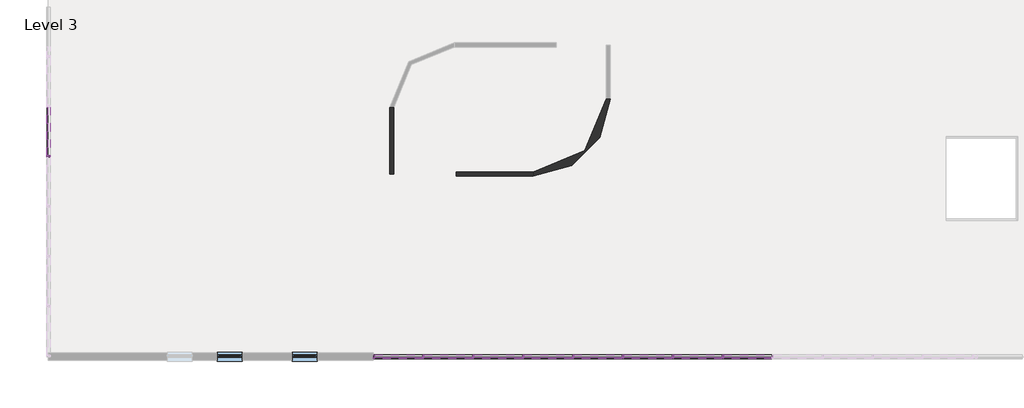
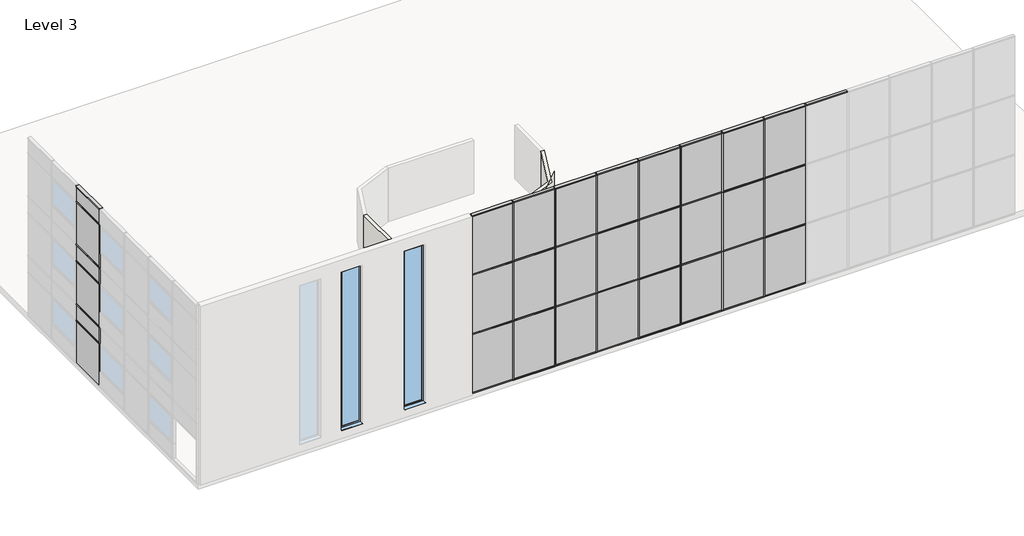
# One storey, part 2 of 5: 69 members, 30 plates, 3 walls, 2 windows.
"""IFC4 building model written with IfcOpenShell, lengths in millimetres."""

import ifcopenshell
import ifcopenshell.guid

model = None  # the IFC model being written
_history = None  # IfcOwnerHistory: only IFC2X3 demands one
_inside = {}  # id of a spatial element -> (the spatial element, [elements in it])
_under = {}  # id of a project, library or spatial element -> (it, [spatial elements below it])
_declared = {}  # id of a project -> (the project, [libraries it declares])
_typed = {}  # id of a type object -> (the type object, [elements of that type])
_made_of = {}  # id of a material, layer set ... -> (it, [elements and type objects made of it])


def new_model(schema):
    """Start an empty IFC model of exactly this schema.

    Asked for "IFC4X3", IfcOpenShell would pick the latest addendum, in which some entities
    have other attributes; the version numbers below select the first issue.
    IFC2X3 requires an IfcOwnerHistory on every rooted entity: one is made here for all.
    """
    global model, _history
    if schema == "IFC4X3":
        model = ifcopenshell.file(schema_version=(4, 3, 0, 0))
    else:
        model = ifcopenshell.file(schema=schema)
    _inside.clear()
    _under.clear()
    _declared.clear()
    _typed.clear()
    _made_of.clear()
    _history = None
    if model.schema == "IFC2X3":
        org = make("IfcOrganization", Name="unknown")
        user = make(
            "IfcPersonAndOrganization",
            ThePerson=make("IfcPerson", FamilyName="unknown"),
            TheOrganization=org,
        )
        app = make(
            "IfcApplication",
            ApplicationDeveloper=org,
            Version="unknown",
            ApplicationFullName="unknown",
            ApplicationIdentifier="unknown",
        )
        _history = make(
            "IfcOwnerHistory",
            OwningUser=user,
            OwningApplication=app,
            ChangeAction="ADDED",
            CreationDate=0,
        )
    return model


def make(cls, **values):
    """One entity of the class cls with the attributes given. An attribute that is None is left unset."""
    return model.create_entity(
        cls, **{name: value for name, value in values.items() if value is not None}
    )


def rooted(cls, **values):
    """An entity with a GlobalId (a new one), such as an element, a storey or a relation."""
    return make(cls, GlobalId=ifcopenshell.guid.new(), OwnerHistory=_history, **values)


def si_unit(unit_type, name, prefix=None):
    """IfcSIUnit, for example si_unit("LENGTHUNIT", "METRE", prefix="MILLI")."""
    return make("IfcSIUnit", UnitType=unit_type, Prefix=prefix, Name=name)


def assignment(units):
    """IfcUnitAssignment: the units of a project."""
    return None if units is None else make("IfcUnitAssignment", Units=units)


def point(xyz):
    """IfcCartesianPoint."""
    return None if xyz is None else make("IfcCartesianPoint", Coordinates=xyz)


def direction(xyz):
    """IfcDirection."""
    return None if xyz is None else make("IfcDirection", DirectionRatios=xyz)


def frame(location, z_axis=None, x_axis=None):
    """IfcAxis2Placement3D, a coordinate frame: its origin and axes. An axis left out is left unset."""
    return make(
        "IfcAxis2Placement3D",
        Location=point(location),
        Axis=direction(z_axis),
        RefDirection=direction(x_axis),
    )


def frame_2d(location, x_axis=None):
    """IfcAxis2Placement2D, a coordinate frame in the plane: its origin and x axis."""
    return make(
        "IfcAxis2Placement2D", Location=point(location), RefDirection=direction(x_axis)
    )


def origin():
    """The frame at (0, 0, 0) with its axes left unset."""
    return frame((0.0, 0.0, 0.0))


def origin_with_axes():
    """The frame at (0, 0, 0) with the z axis (0, 0, 1) and the x axis (1, 0, 0) written out."""
    return frame((0.0, 0.0, 0.0), z_axis=(0.0, 0.0, 1.0), x_axis=(1.0, 0.0, 0.0))


def place(relative_to, where):
    """IfcLocalPlacement: puts the frame where relative to a parent placement (None: the world)."""
    return make(
        "IfcLocalPlacement", PlacementRelTo=relative_to, RelativePlacement=where
    )


def context(
    kind, dimensions, precision=None, world=None, true_north=None, identifier=None
):
    """IfcGeometricRepresentationContext, for example the 3D "Model" context."""
    return make(
        "IfcGeometricRepresentationContext",
        ContextIdentifier=identifier,
        ContextType=kind,
        CoordinateSpaceDimension=dimensions,
        Precision=precision,
        WorldCoordinateSystem=world,
        TrueNorth=true_north,
    )


def project(units=None, contexts=None):
    """IfcProject with its units and contexts."""
    return rooted(
        "IfcProject",
        Name="project",
        RepresentationContexts=contexts,
        UnitsInContext=assignment(units),
    )


def spatial(cls, under=None, at=None, **own):
    """A site, building, storey or space (cls), placed at a placement, below another one or the project."""
    s = rooted(cls, ObjectPlacement=at, **own)
    if under is not None:
        _under.setdefault(under.id(), (under, []))[1].append(s)
    return s


def polyline(points):
    """IfcPolyline through the points."""
    return make("IfcPolyline", Points=[point(p) for p in points])


def circle_curve(where, radius):
    """IfcCircle in the frame where."""
    return make("IfcCircle", Position=where, Radius=radius)


def trimmed(basis, trim1, trim2, sense, master):
    """IfcTrimmedCurve: the piece of a basis curve between two trims."""
    return make(
        "IfcTrimmedCurve",
        BasisCurve=basis,
        Trim1=trim1,
        Trim2=trim2,
        SenseAgreement=sense,
        MasterRepresentation=master,
    )


def segment(curve, same_sense, transition):
    """IfcCompositeCurveSegment."""
    return make(
        "IfcCompositeCurveSegment",
        Transition=transition,
        SameSense=same_sense,
        ParentCurve=curve,
    )


def composite_curve(segments, self_intersect=None):
    """IfcCompositeCurve: segments joined end to end."""
    return make("IfcCompositeCurve", Segments=segments, SelfIntersect=self_intersect)


def outline(outer, holes=None, kind="AREA"):
    """IfcArbitraryClosedProfileDef: a profile drawn as a closed curve; with holes, ...WithVoids."""
    if holes is None:
        return make("IfcArbitraryClosedProfileDef", ProfileType=kind, OuterCurve=outer)
    return make(
        "IfcArbitraryProfileDefWithVoids",
        ProfileType=kind,
        OuterCurve=outer,
        InnerCurves=holes,
    )


def extrude(swept, where, along, depth):
    """IfcExtrudedAreaSolid: the profile swept, set in the frame where, extruded along a direction by depth."""
    return make(
        "IfcExtrudedAreaSolid",
        SweptArea=swept,
        Position=where,
        ExtrudedDirection=direction(along),
        Depth=depth,
    )


def faces_of(points, faces, orient=None, outer=None):
    """IfcFace entities. A face is a list of loops; a loop is a list of indices into points, from 0.

    orient and outer hold one flag for each loop. By default every Orientation is true, the
    first loop of a face is its IfcFaceOuterBound and the others are IfcFaceBound.
    """
    made = []
    for i, loops in enumerate(faces):
        bounds = []
        for j, loop in enumerate(loops):
            is_outer = j == 0 if outer is None else outer[i][j]
            bounds.append(
                make(
                    "IfcFaceOuterBound" if is_outer else "IfcFaceBound",
                    Bound=make("IfcPolyLoop", Polygon=[points[k] for k in loop]),
                    Orientation=True if orient is None else orient[i][j],
                )
            )
        made.append(make("IfcFace", Bounds=bounds))
    return made


def faceted_brep(points, faces, orient=None, outer=None, voids=None):
    """IfcFacetedBrep: a solid bounded by flat faces; with voids (closed shells), ...WithVoids."""
    shared = [point(p) for p in points]
    hull = make("IfcClosedShell", CfsFaces=faces_of(shared, faces, orient, outer))
    if voids is None:
        return make("IfcFacetedBrep", Outer=hull)
    return make(
        "IfcFacetedBrepWithVoids",
        Outer=hull,
        Voids=[
            make(cls, CfsFaces=faces_of(shared, fs, o, b)) for cls, fs, o, b in voids
        ],
    )


def shape(context_of_items, identifier, shape_type, items):
    """IfcShapeRepresentation: the items that make up one representation, for example the "Body"."""
    return make(
        "IfcShapeRepresentation",
        ContextOfItems=context_of_items,
        RepresentationIdentifier=identifier,
        RepresentationType=shape_type,
        Items=items,
    )


def source(mapping_origin, context_of_items, identifier, shape_type, items):
    """IfcRepresentationMap: a shape defined once, which mapped items show again and again."""
    return make(
        "IfcRepresentationMap",
        MappingOrigin=mapping_origin,
        MappedRepresentation=shape(context_of_items, identifier, shape_type, items),
    )


def transform(
    local_origin,
    x_axis=None,
    y_axis=None,
    z_axis=None,
    scale=None,
    scale2=None,
    scale3=None,
    uniform=True,
):
    """IfcCartesianTransformationOperator3D, or its non-uniform kind. x_axis, y_axis, z_axis: its Axis1, 2, 3."""
    if uniform:
        return make(
            "IfcCartesianTransformationOperator3D",
            Axis1=direction(x_axis),
            Axis2=direction(y_axis),
            LocalOrigin=point(local_origin),
            Scale=scale,
            Axis3=direction(z_axis),
        )
    return make(
        "IfcCartesianTransformationOperator3DnonUniform",
        Axis1=direction(x_axis),
        Axis2=direction(y_axis),
        LocalOrigin=point(local_origin),
        Scale=scale,
        Axis3=direction(z_axis),
        Scale2=scale2,
        Scale3=scale3,
    )


def mapped(mapping_source, mapping_target):
    """IfcMappedItem: shows the shape of a source again, moved by a transform."""
    return make(
        "IfcMappedItem", MappingSource=mapping_source, MappingTarget=mapping_target
    )


def made_of(thing, what):
    """Note that an element or type object is made of a material, layer set ...; save() writes the relation."""
    if what is not None:
        _made_of.setdefault(what.id(), (what, []))[1].append(thing)
    return thing


def element(
    cls,
    number,
    at=None,
    inside=None,
    cuts=None,
    type_object=None,
    material=None,
    context=None,
    identifier="Body",
    shape_type=None,
    held_by="IfcProductDefinitionShape",
    body=None,
    shapes=None,
    **own,
):
    """One element of the class cls, such as IfcWall. Its Tag is "e" and its number.

    at: its placement. inside: the storey or other place that contains it. cuts: it is an
    opening in that element (IfcRelVoidsElement). A single representation is given by context,
    identifier, shape_type and body (its items); several are given by shapes. held_by: the class
    of the entity that holds the representations. save() writes the other relations.
    """
    e = rooted(cls, Tag="e%d" % number, ObjectPlacement=at, **own)
    if body is not None:
        shapes = [shape(context, identifier, shape_type, body)]
    if shapes is not None:
        e.Representation = make(held_by, Representations=shapes)
    if inside is not None:
        _inside.setdefault(inside.id(), (inside, []))[1].append(e)
    if cuts is not None:
        rooted(
            "IfcRelVoidsElement", RelatingBuildingElement=cuts, RelatedOpeningElement=e
        )
    if type_object is not None:
        _typed.setdefault(type_object.id(), (type_object, []))[1].append(e)
    return made_of(e, material)


def aggregate(whole, parts):
    """IfcRelAggregates: a whole, such as a stair, and the parts it consists of."""
    return rooted("IfcRelAggregates", RelatingObject=whole, RelatedObjects=parts)


def save(model, path):
    """Write the relations noted so far, then the file.

    IfcRelAggregates (storeys below a building ...), IfcRelContainedInSpatialStructure (elements
    in a storey), IfcRelDefinesByType, IfcRelAssociatesMaterial and IfcRelDeclares: one each for
    every whole, place, type object, material and project.
    """
    for whole, parts in _under.values():
        aggregate(whole, parts)
    for where, things in _inside.values():
        rooted(
            "IfcRelContainedInSpatialStructure",
            RelatedElements=things,
            RelatingStructure=where,
        )
    for kind, things in _typed.values():
        rooted("IfcRelDefinesByType", RelatedObjects=things, RelatingType=kind)
    for what, things in _made_of.values():
        rooted("IfcRelAssociatesMaterial", RelatedObjects=things, RelatingMaterial=what)
    for by, libraries in _declared.values():
        rooted("IfcRelDeclares", RelatingContext=by, RelatedDefinitions=libraries)
    model.write(path)


def rectangular_mullion_50_x_150mm_f1645b81(model_context):
    return source(origin(), model_context, "Body", "SweptSolid", [
        extrude(outline(polyline([(25.0, 75.0), (25.0, -75.0), (-25.0, -75.0), (-25.0, 75.0), (25.0, 75.0)])), frame((0.0, 0.0, -1950.0000003), z_axis=(0.0, 0.0, 1.0), x_axis=(1.0, 0.0, 0.0)), (0.0, 0.0, 1.0), 1950.0000003),
    ])


def rectangular_mullion_50_x_150mm_0967fd3c(model_context):
    return source(origin(), model_context, "Body", "SweptSolid", [
        extrude(outline(polyline([(0.0, 75.0), (0.0, -75.0), (-50.0, -75.0), (-50.0, 75.0), (0.0, 75.0)])), frame((0.0, 0.0, -1950.0000003), z_axis=(0.0, 0.0, 1.0), x_axis=(1.0, 0.0, 0.0)), (0.0, 0.0, 1.0), 1950.0000003),
    ])


def rectangular_mullion_50_x_150mm_6270d9f9(model_context):
    return source(origin(), model_context, "Body", "SweptSolid", [
        extrude(outline(polyline([(25.0, 75.0), (25.0, -75.0), (-25.0, -75.0), (-25.0, 75.0), (25.0, 75.0)])), frame((0.0, 0.0, -775.0), z_axis=(0.0, 0.0, 1.0), x_axis=(1.0, 0.0, 0.0)), (0.0, 0.0, 1.0), 775.0),
    ])


def rectangular_mullion_50_x_150mm_80d7b263(model_context):
    return source(origin(), model_context, "Body", "SweptSolid", [
        extrude(outline(polyline([(25.0, 75.0), (25.0, -75.0), (-25.0, -75.0), (-25.0, 75.0), (25.0, 75.0)])), frame((0.0, 0.0, -1400.0), z_axis=(0.0, 0.0, 1.0), x_axis=(1.0, 0.0, 0.0)), (0.0, 0.0, 1.0), 1400.0),
    ])


def rectangular_mullion_50_x_150mm_9c26cac3(model_context):
    return source(origin(), model_context, "Body", "SweptSolid", [
        extrude(outline(polyline([(25.0, 75.0), (25.0, -75.0), (-25.0, -75.0), (-25.0, 75.0), (25.0, 75.0)])), frame((0.0, 0.0, -825.0), z_axis=(0.0, 0.0, 1.0), x_axis=(1.0, 0.0, 0.0)), (0.0, 0.0, 1.0), 825.0),
    ])


def rectangular_mullion_50_x_150mm_6c7cb899(model_context):
    return source(origin(), model_context, "Body", "SweptSolid", [
        extrude(outline(polyline([(25.0, 75.0), (25.0, -75.0), (-25.0, -75.0), (-25.0, 75.0), (25.0, 75.0)])), frame((0.0, 0.0, -3000.0), z_axis=(0.0, 0.0, 1.0), x_axis=(1.0, 0.0, 0.0)), (0.0, 0.0, 1.0), 3000.0),
    ])


def rectangular_mullion_50_x_150mm_68c91185(model_context):
    return source(origin(), model_context, "Body", "SweptSolid", [
        extrude(outline(polyline([(0.0, 75.0), (0.0, -75.0), (-50.0, -75.0), (-50.0, 75.0), (0.0, 75.0)])), frame((0.0, 0.0, -3000.0), z_axis=(0.0, 0.0, 1.0), x_axis=(1.0, 0.0, 0.0)), (0.0, 0.0, 1.0), 3000.0),
    ])


def rectangular_mullion_50_x_150mm_7828da58(model_context):
    return source(origin(), model_context, "Body", "SweptSolid", [
        extrude(outline(polyline([(0.0, 75.0), (0.0, -75.0), (-50.0, -75.0), (-50.0, 75.0), (0.0, 75.0)])), frame((0.0, 0.0, -1923.3666669), z_axis=(0.0, 0.0, 1.0), x_axis=(1.0, 0.0, 0.0)), (0.0, 0.0, 1.0), 1923.3666669),
    ])


def rectangular_mullion_50_x_150mm_2c1a111c(model_context):
    return source(origin(), model_context, "Body", "SweptSolid", [
        extrude(outline(polyline([(0.0, 75.0), (0.0, -75.0), (-50.0, -75.0), (-50.0, 75.0), (0.0, 75.0)])), frame((0.0, 0.0, -1948.3666666), z_axis=(0.0, 0.0, 1.0), x_axis=(1.0, 0.0, 0.0)), (0.0, 0.0, 1.0), 1948.3666666),
    ])


def rectangular_mullion_50_x_150mm_6ba4331c(model_context):
    return source(origin(), model_context, "Body", "SweptSolid", [
        extrude(outline(polyline([(25.0, 75.0), (25.0, -75.0), (-25.0, -75.0), (-25.0, 75.0), (25.0, 75.0)])), frame((0.0, 0.0, -1923.3666669), z_axis=(0.0, 0.0, 1.0), x_axis=(1.0, 0.0, 0.0)), (0.0, 0.0, 1.0), 1923.3666669),
    ])


def rectangular_mullion_50_x_150mm_825cde95(model_context):
    return source(origin(), model_context, "Body", "SweptSolid", [
        extrude(outline(polyline([(25.0, 75.0), (25.0, -75.0), (-25.0, -75.0), (-25.0, 75.0), (25.0, 75.0)])), frame((0.0, 0.0, -1948.3666666), z_axis=(0.0, 0.0, 1.0), x_axis=(1.0, 0.0, 0.0)), (0.0, 0.0, 1.0), 1948.3666666),
    ])


def system_panel_glazed_1e38db9b(model_context):
    return source(origin(), model_context, "Body", "SweptSolid", [
        extrude(outline(polyline([(0.0, -975.0000002), (0.0, 975.0000002), (750.0, 975.0000002), (2125.0, 975.0000002), (2125.0, -975.0000002), (750.0, -975.0000002), (0.0, -975.0000002)])), frame((0.0, 24.5, 0.0), z_axis=(0.0, 1.0, 0.0), x_axis=(0.0, 0.0, 1.0)), (0.0, 0.0, 1.0), 25.0),
    ])


def system_panel_glazed_bc1ebc0c(model_context):
    return source(origin(), model_context, "Body", "SweptSolid", [
        extrude(outline(polyline([(975.0000002, 24.5), (-975.0000002, 24.5), (-975.0000002, 49.5), (975.0000002, 49.5), (975.0000002, 24.5)])), origin_with_axes(), (0.0, 0.0, 1.0), 725.0),
    ])


def system_panel_glazed_d82c9dbb(model_context):
    return source(origin(), model_context, "Body", "SweptSolid", [
        extrude(outline(polyline([(975.0000002, 24.5), (-975.0000002, 24.5), (-975.0000002, 49.5), (975.0000002, 49.5), (975.0000002, 24.5)])), origin_with_axes(), (0.0, 0.0, 1.0), 775.0),
    ])


def system_panel_glazed_19a6ddb1(model_context):
    return source(origin(), model_context, "Body", "SweptSolid", [
        extrude(outline(polyline([(961.6833335, 24.5), (-961.6833335, 24.5), (-961.6833335, 49.5), (961.6833335, 49.5), (961.6833335, 24.5)])), origin_with_axes(), (0.0, 0.0, 1.0), 2925.0),
    ])


def system_panel_glazed_e38ee6be(model_context):
    return source(origin(), model_context, "Body", "SweptSolid", [
        extrude(outline(polyline([(974.1833333, 24.5), (-974.1833333, 24.5), (-974.1833333, 49.5), (974.1833333, 49.5), (974.1833333, 24.5)])), origin_with_axes(), (0.0, 0.0, 1.0), 2925.0),
    ])


def system_panel_glazed_cab7de13(model_context):
    return source(origin(), model_context, "Body", "SweptSolid", [
        extrude(outline(polyline([(961.6833335, 24.5), (-961.6833335, 24.5), (-961.6833335, 49.5), (961.6833335, 49.5), (961.6833335, 24.5)])), origin_with_axes(), (0.0, 0.0, 1.0), 2950.0),
    ])


def system_panel_glazed_2cf92cf8(model_context):
    return source(origin(), model_context, "Body", "SweptSolid", [
        extrude(outline(polyline([(974.1833333, 24.5), (-974.1833333, 24.5), (-974.1833333, 49.5), (974.1833333, 49.5), (974.1833333, 24.5)])), origin_with_axes(), (0.0, 0.0, 1.0), 2950.0),
    ])


def window_variable_standard_9eb8f332(model_context):
    return source(origin(), model_context, "Body", "SolidModel", [
        extrude(outline(polyline([(9000.0, 500.0), (9000.0, -500.0), (1000.0, -500.0), (1000.0, 500.0), (9000.0, 500.0)]), holes=[polyline([(8920.0, 440.0), (1080.0, 440.0), (1080.0, -440.0), (8920.0, -440.0), (8920.0, 440.0)])]), frame((0.0, -70.0, 0.0), z_axis=(0.0, 1.0, 0.0), x_axis=(0.0, 0.0, 1.0)), (0.0, 0.0, 1.0), 60.0),
        faceted_brep([(470.0, -10.0, 8950.0), (470.0, -10.0, 1050.0), (470.0, 20.0, 1050.0), (470.0, 20.0, 8950.0), (-470.0, 20.0, 1050.0), (-470.0, 20.0, 8950.0), (410.0, 20.0, 1110.0), (410.0, 20.0, 8890.0), (-410.0, 20.0, 8890.0), (-410.0, 20.0, 1110.0), (-470.0, -10.0, 1050.0), (-470.0, -10.0, 8950.0), (440.0, -10.0, 8920.0), (440.0, -10.0, 1080.0), (-440.0, -10.0, 1080.0), (-440.0, -10.0, 8920.0), (440.0, -40.0, 8920.0), (440.0, -40.0, 1080.0), (-440.0, -40.0, 1080.0), (-440.0, -40.0, 8920.0), (410.0, -40.0, 8890.0), (410.0, -40.0, 1110.0), (-410.0, -40.0, 1110.0), (-410.0, -40.0, 8890.0)], [[[0, 1, 2, 3]], [[3, 2, 4, 5], [6, 7, 8, 9]], [[1, 10, 4, 2]], [[1, 0, 11, 10], [12, 13, 14, 15]], [[16, 17, 13, 12]], [[17, 18, 14, 13]], [[17, 16, 19, 18], [20, 21, 22, 23]], [[7, 6, 21, 20]], [[6, 9, 22, 21]], [[10, 11, 5, 4]], [[18, 19, 15, 14]], [[9, 8, 23, 22]], [[11, 0, 3, 5]], [[19, 16, 12, 15]], [[8, 7, 20, 23]]]),
        extrude(outline(polyline([(-500.0, 180.0), (500.0, 180.0), (500.0, -10.0), (-500.0, -10.0), (-500.0, 180.0)])), frame((0.0, 0.0, 1005.0), z_axis=(0.0, 0.0, 1.0), x_axis=(1.0, 0.0, 0.0)), (0.0, 0.0, 1.0), 15.0),
        extrude(outline(polyline([(-80.0221543, 1020.0), (-70.0, 1020.0), (-70.0, 1018.0), (-79.8240723, 1018.0), (-178.0, 998.3604634), (-178.0, 990.0), (-180.0, 990.0), (-180.0, 1000.0), (-80.0221543, 1020.0)])), frame((-500.0, 0.0, 0.0), z_axis=(1.0, 0.0, 0.0), x_axis=(0.0, 1.0, 0.0)), (0.0, 0.0, 1.0), 1000.0),
        extrude(outline(polyline([(410.0, 5.0), (410.0, -25.0), (-410.0, -25.0), (-410.0, 5.0), (410.0, 5.0)])), frame((0.0, 0.0, 1110.0), z_axis=(0.0, 0.0, 1.0), x_axis=(1.0, 0.0, 0.0)), (0.0, 0.0, 1.0), 7780.0),
    ])


model = new_model("IFC4")

# Units and contexts
model_context = context("Model", 3, world=origin())
ifc_project = project(units=[si_unit("LENGTHUNIT", "METRE", prefix="MILLI")], contexts=[model_context])

# Site, building, storey
site = spatial("IfcSite", under=ifc_project)
building = spatial("IfcBuilding", under=site)
storey = spatial("IfcBuildingStorey", under=building, Name="Level 3", Elevation=6000.0)

# Members
placement = place(None, origin())
rectangular_mullion_50_x_150mm_shape = rectangular_mullion_50_x_150mm_f1645b81(model_context)
element("IfcMember", 1, ObjectType="Rectangular Mullion : 50 x 150mm", at=placement, inside=storey, context=model_context, shape_type="MappedRepresentation", body=[
    mapped(rectangular_mullion_50_x_150mm_shape, transform((-6732.0028633, -1.2422767, 14200.0), x_axis=(0.0, 0.0, 1.0), y_axis=(1.0, 0.0, 0.0), z_axis=(0.0, 1.0, 0.0))),
])
element("IfcMember", 2, ObjectType="Rectangular Mullion : 50 x 150mm", at=placement, inside=storey, context=model_context, shape_type="MappedRepresentation", body=[
    mapped(rectangular_mullion_50_x_150mm_shape, transform((-6732.0028633, -1.2422767, 9025.0), x_axis=(0.0, 0.0, 1.0), y_axis=(1.0, 0.0, 0.0), z_axis=(0.0, 1.0, 0.0))),
])
element("IfcMember", 3, ObjectType="Rectangular Mullion : 50 x 150mm", at=placement, inside=storey, context=model_context, shape_type="MappedRepresentation", body=[
    mapped(rectangular_mullion_50_x_150mm_shape, transform((-6732.0028633, -1.2422767, 12025.0), x_axis=(0.0, 0.0, 1.0), y_axis=(1.0, 0.0, 0.0), z_axis=(0.0, 1.0, 0.0))),
])
element("IfcMember", 4, ObjectType="Rectangular Mullion : 50 x 150mm", at=placement, inside=storey, context=model_context, shape_type="MappedRepresentation", body=[
    mapped(rectangular_mullion_50_x_150mm_shape, transform((-6732.0028633, -1.2422767, 11200.0), x_axis=(0.0, 0.0, 1.0), y_axis=(1.0, 0.0, 0.0), z_axis=(0.0, 1.0, 0.0))),
])
element("IfcMember", 5, ObjectType="Rectangular Mullion : 50 x 150mm", at=placement, inside=storey, context=model_context, shape_type="MappedRepresentation", body=[
    mapped(rectangular_mullion_50_x_150mm_shape, transform((-6732.0028633, -1.2422767, 8200.0), x_axis=(0.0, 0.0, 1.0), y_axis=(1.0, 0.0, 0.0), z_axis=(0.0, 1.0, 0.0))),
])
rectangular_mullion_50_x_150mm_2_shape = rectangular_mullion_50_x_150mm_0967fd3c(model_context)
element("IfcMember", 6, ObjectType="Rectangular Mullion : 50 x 150mm", at=placement, inside=storey, context=model_context, shape_type="MappedRepresentation", body=[
    mapped(rectangular_mullion_50_x_150mm_2_shape, transform((-6732.0028633, -1.2422767, 15000.0), x_axis=(0.0, 0.0, 1.0), y_axis=(1.0, 0.0, 0.0), z_axis=(0.0, 1.0, 0.0))),
])
rectangular_mullion_50_x_150mm_3_shape = rectangular_mullion_50_x_150mm_6270d9f9(model_context)
element("IfcMember", 7, ObjectType="Rectangular Mullion : 50 x 150mm", at=placement, inside=storey, context=model_context, shape_type="MappedRepresentation", body=[
    mapped(rectangular_mullion_50_x_150mm_3_shape, transform((-6732.0028633, -1976.2422767, 12025.0), x_axis=(0.0, 1.0, 0.0), y_axis=(1.0, 0.0, 0.0), z_axis=(0.0, 0.0, -1.0))),
])
rectangular_mullion_50_x_150mm_4_shape = rectangular_mullion_50_x_150mm_80d7b263(model_context)
element("IfcMember", 8, ObjectType="Rectangular Mullion : 50 x 150mm", at=placement, inside=storey, context=model_context, shape_type="MappedRepresentation", body=[
    mapped(rectangular_mullion_50_x_150mm_4_shape, transform((-6732.0028633, -1976.2422767, 12800.0), x_axis=(0.0, 1.0, 0.0), y_axis=(1.0, 0.0, 0.0), z_axis=(0.0, 0.0, -1.0))),
])
element("IfcMember", 9, ObjectType="Rectangular Mullion : 50 x 150mm", at=placement, inside=storey, context=model_context, shape_type="MappedRepresentation", body=[
    mapped(rectangular_mullion_50_x_150mm_4_shape, transform((-6732.0028633, -1976.2422767, 9800.0), x_axis=(0.0, 1.0, 0.0), y_axis=(1.0, 0.0, 0.0), z_axis=(0.0, 0.0, -1.0))),
])
element("IfcMember", 10, ObjectType="Rectangular Mullion : 50 x 150mm", at=placement, inside=storey, context=model_context, shape_type="MappedRepresentation", body=[
    mapped(rectangular_mullion_50_x_150mm_4_shape, transform((-6732.0028633, -1976.2422767, 6800.0), x_axis=(0.0, 1.0, 0.0), y_axis=(1.0, 0.0, 0.0), z_axis=(0.0, 0.0, -1.0))),
])
rectangular_mullion_50_x_150mm_5_shape = rectangular_mullion_50_x_150mm_9c26cac3(model_context)
element("IfcMember", 11, ObjectType="Rectangular Mullion : 50 x 150mm", at=placement, inside=storey, context=model_context, shape_type="MappedRepresentation", body=[
    mapped(rectangular_mullion_50_x_150mm_5_shape, transform((-6732.0028633, -1976.2422767, 11200.0), x_axis=(0.0, 1.0, 0.0), y_axis=(1.0, 0.0, 0.0), z_axis=(0.0, 0.0, -1.0))),
])
element("IfcMember", 12, ObjectType="Rectangular Mullion : 50 x 150mm", at=placement, inside=storey, context=model_context, shape_type="MappedRepresentation", body=[
    mapped(rectangular_mullion_50_x_150mm_5_shape, transform((-6732.0028633, -1976.2422767, 8200.0), x_axis=(0.0, 1.0, 0.0), y_axis=(1.0, 0.0, 0.0), z_axis=(0.0, 0.0, -1.0))),
])
rectangular_mullion_50_x_150mm_6_shape = rectangular_mullion_50_x_150mm_6c7cb899(model_context)
element("IfcMember", 13, ObjectType="Rectangular Mullion : 50 x 150mm", at=placement, inside=storey, context=model_context, shape_type="MappedRepresentation", body=[
    mapped(rectangular_mullion_50_x_150mm_6_shape, transform((20256.5638033, -10001.242277, 6000.0), x_axis=(-1.0, 0.0, 0.0), y_axis=(0.0, 1.0, 0.0), z_axis=(0.0, 0.0, -1.0))),
])
element("IfcMember", 14, ObjectType="Rectangular Mullion : 50 x 150mm", at=placement, inside=storey, context=model_context, shape_type="MappedRepresentation", body=[
    mapped(rectangular_mullion_50_x_150mm_6_shape, transform((18258.1971367, -10001.242277, 6000.0), x_axis=(-1.0, 0.0, 0.0), y_axis=(0.0, 1.0, 0.0), z_axis=(0.0, 0.0, -1.0))),
])
element("IfcMember", 15, ObjectType="Rectangular Mullion : 50 x 150mm", at=placement, inside=storey, context=model_context, shape_type="MappedRepresentation", body=[
    mapped(rectangular_mullion_50_x_150mm_6_shape, transform((16259.8304701, -10001.242277, 6000.0), x_axis=(-1.0, 0.0, 0.0), y_axis=(0.0, 1.0, 0.0), z_axis=(0.0, 0.0, -1.0))),
])
element("IfcMember", 16, ObjectType="Rectangular Mullion : 50 x 150mm", at=placement, inside=storey, context=model_context, shape_type="MappedRepresentation", body=[
    mapped(rectangular_mullion_50_x_150mm_6_shape, transform((14261.4638035, -10001.242277, 6000.0), x_axis=(-1.0, 0.0, 0.0), y_axis=(0.0, 1.0, 0.0), z_axis=(0.0, 0.0, -1.0))),
])
element("IfcMember", 17, ObjectType="Rectangular Mullion : 50 x 150mm", at=placement, inside=storey, context=model_context, shape_type="MappedRepresentation", body=[
    mapped(rectangular_mullion_50_x_150mm_6_shape, transform((12263.0971368, -10001.242277, 6000.0), x_axis=(-1.0, 0.0, 0.0), y_axis=(0.0, 1.0, 0.0), z_axis=(0.0, 0.0, -1.0))),
])
element("IfcMember", 18, ObjectType="Rectangular Mullion : 50 x 150mm", at=placement, inside=storey, context=model_context, shape_type="MappedRepresentation", body=[
    mapped(rectangular_mullion_50_x_150mm_6_shape, transform((10264.7304702, -10001.242277, 6000.0), x_axis=(-1.0, 0.0, 0.0), y_axis=(0.0, 1.0, 0.0), z_axis=(0.0, 0.0, -1.0))),
])
element("IfcMember", 19, ObjectType="Rectangular Mullion : 50 x 150mm", at=placement, inside=storey, context=model_context, shape_type="MappedRepresentation", body=[
    mapped(rectangular_mullion_50_x_150mm_6_shape, transform((8266.3638036, -10001.242277, 6000.0), x_axis=(-1.0, 0.0, 0.0), y_axis=(0.0, 1.0, 0.0), z_axis=(0.0, 0.0, -1.0))),
])
rectangular_mullion_50_x_150mm_7_shape = rectangular_mullion_50_x_150mm_68c91185(model_context)
element("IfcMember", 20, ObjectType="Rectangular Mullion : 50 x 150mm", at=placement, inside=storey, context=model_context, shape_type="MappedRepresentation", body=[
    mapped(rectangular_mullion_50_x_150mm_7_shape, transform((6267.9971367, -10001.242277, 6000.0), x_axis=(-1.0, 0.0, 0.0), y_axis=(0.0, 1.0, 0.0), z_axis=(0.0, 0.0, -1.0))),
])
rectangular_mullion_50_x_150mm_8_shape = rectangular_mullion_50_x_150mm_7828da58(model_context)
element("IfcMember", 21, ObjectType="Rectangular Mullion : 50 x 150mm", at=placement, inside=storey, context=model_context, shape_type="MappedRepresentation", body=[
    mapped(rectangular_mullion_50_x_150mm_8_shape, transform((6317.9971367, -10001.242277, 15000.0), x_axis=(0.0, 0.0, 1.0), y_axis=(0.0, 1.0, 0.0), z_axis=(-1.0, 0.0, 0.0))),
])
element("IfcMember", 22, ObjectType="Rectangular Mullion : 50 x 150mm", at=placement, inside=storey, context=model_context, shape_type="MappedRepresentation", body=[
    mapped(rectangular_mullion_50_x_150mm_8_shape, transform((8241.3638036, -10001.242277, 6000.0), x_axis=(0.0, 0.0, -1.0), y_axis=(0.0, 1.0, 0.0), z_axis=(1.0, 0.0, 0.0))),
])
rectangular_mullion_50_x_150mm_9_shape = rectangular_mullion_50_x_150mm_2c1a111c(model_context)
element("IfcMember", 23, ObjectType="Rectangular Mullion : 50 x 150mm", at=placement, inside=storey, context=model_context, shape_type="MappedRepresentation", body=[
    mapped(rectangular_mullion_50_x_150mm_9_shape, transform((22279.93047, -10001.242277, 15000.0), x_axis=(0.0, 0.0, 1.0), y_axis=(0.0, 1.0, 0.0), z_axis=(-1.0, 0.0, 0.0))),
])
element("IfcMember", 24, ObjectType="Rectangular Mullion : 50 x 150mm", at=placement, inside=storey, context=model_context, shape_type="MappedRepresentation", body=[
    mapped(rectangular_mullion_50_x_150mm_9_shape, transform((20281.5638033, -10001.242277, 15000.0), x_axis=(0.0, 0.0, 1.0), y_axis=(0.0, 1.0, 0.0), z_axis=(-1.0, 0.0, 0.0))),
])
element("IfcMember", 25, ObjectType="Rectangular Mullion : 50 x 150mm", at=placement, inside=storey, context=model_context, shape_type="MappedRepresentation", body=[
    mapped(rectangular_mullion_50_x_150mm_9_shape, transform((18283.1971367, -10001.242277, 15000.0), x_axis=(0.0, 0.0, 1.0), y_axis=(0.0, 1.0, 0.0), z_axis=(-1.0, 0.0, 0.0))),
])
element("IfcMember", 26, ObjectType="Rectangular Mullion : 50 x 150mm", at=placement, inside=storey, context=model_context, shape_type="MappedRepresentation", body=[
    mapped(rectangular_mullion_50_x_150mm_9_shape, transform((16284.8304701, -10001.242277, 15000.0), x_axis=(0.0, 0.0, 1.0), y_axis=(0.0, 1.0, 0.0), z_axis=(-1.0, 0.0, 0.0))),
])
element("IfcMember", 27, ObjectType="Rectangular Mullion : 50 x 150mm", at=placement, inside=storey, context=model_context, shape_type="MappedRepresentation", body=[
    mapped(rectangular_mullion_50_x_150mm_9_shape, transform((14286.4638035, -10001.242277, 15000.0), x_axis=(0.0, 0.0, 1.0), y_axis=(0.0, 1.0, 0.0), z_axis=(-1.0, 0.0, 0.0))),
])
element("IfcMember", 28, ObjectType="Rectangular Mullion : 50 x 150mm", at=placement, inside=storey, context=model_context, shape_type="MappedRepresentation", body=[
    mapped(rectangular_mullion_50_x_150mm_9_shape, transform((12288.0971368, -10001.242277, 15000.0), x_axis=(0.0, 0.0, 1.0), y_axis=(0.0, 1.0, 0.0), z_axis=(-1.0, 0.0, 0.0))),
])
element("IfcMember", 29, ObjectType="Rectangular Mullion : 50 x 150mm", at=placement, inside=storey, context=model_context, shape_type="MappedRepresentation", body=[
    mapped(rectangular_mullion_50_x_150mm_9_shape, transform((10289.7304702, -10001.242277, 15000.0), x_axis=(0.0, 0.0, 1.0), y_axis=(0.0, 1.0, 0.0), z_axis=(-1.0, 0.0, 0.0))),
])
element("IfcMember", 30, ObjectType="Rectangular Mullion : 50 x 150mm", at=placement, inside=storey, context=model_context, shape_type="MappedRepresentation", body=[
    mapped(rectangular_mullion_50_x_150mm_9_shape, transform((8291.3638036, -10001.242277, 15000.0), x_axis=(0.0, 0.0, 1.0), y_axis=(0.0, 1.0, 0.0), z_axis=(-1.0, 0.0, 0.0))),
])
element("IfcMember", 31, ObjectType="Rectangular Mullion : 50 x 150mm", at=placement, inside=storey, context=model_context, shape_type="MappedRepresentation", body=[
    mapped(rectangular_mullion_50_x_150mm_9_shape, transform((22229.93047, -10001.242277, 6000.0), x_axis=(0.0, 0.0, -1.0), y_axis=(0.0, 1.0, 0.0), z_axis=(1.0, 0.0, 0.0))),
])
element("IfcMember", 32, ObjectType="Rectangular Mullion : 50 x 150mm", at=placement, inside=storey, context=model_context, shape_type="MappedRepresentation", body=[
    mapped(rectangular_mullion_50_x_150mm_9_shape, transform((20231.5638033, -10001.242277, 6000.0), x_axis=(0.0, 0.0, -1.0), y_axis=(0.0, 1.0, 0.0), z_axis=(1.0, 0.0, 0.0))),
])
element("IfcMember", 33, ObjectType="Rectangular Mullion : 50 x 150mm", at=placement, inside=storey, context=model_context, shape_type="MappedRepresentation", body=[
    mapped(rectangular_mullion_50_x_150mm_9_shape, transform((18233.1971367, -10001.242277, 6000.0), x_axis=(0.0, 0.0, -1.0), y_axis=(0.0, 1.0, 0.0), z_axis=(1.0, 0.0, 0.0))),
])
element("IfcMember", 34, ObjectType="Rectangular Mullion : 50 x 150mm", at=placement, inside=storey, context=model_context, shape_type="MappedRepresentation", body=[
    mapped(rectangular_mullion_50_x_150mm_9_shape, transform((16234.8304701, -10001.242277, 6000.0), x_axis=(0.0, 0.0, -1.0), y_axis=(0.0, 1.0, 0.0), z_axis=(1.0, 0.0, 0.0))),
])
element("IfcMember", 35, ObjectType="Rectangular Mullion : 50 x 150mm", at=placement, inside=storey, context=model_context, shape_type="MappedRepresentation", body=[
    mapped(rectangular_mullion_50_x_150mm_9_shape, transform((14236.4638035, -10001.242277, 6000.0), x_axis=(0.0, 0.0, -1.0), y_axis=(0.0, 1.0, 0.0), z_axis=(1.0, 0.0, 0.0))),
])
element("IfcMember", 36, ObjectType="Rectangular Mullion : 50 x 150mm", at=placement, inside=storey, context=model_context, shape_type="MappedRepresentation", body=[
    mapped(rectangular_mullion_50_x_150mm_9_shape, transform((12238.0971368, -10001.242277, 6000.0), x_axis=(0.0, 0.0, -1.0), y_axis=(0.0, 1.0, 0.0), z_axis=(1.0, 0.0, 0.0))),
])
element("IfcMember", 37, ObjectType="Rectangular Mullion : 50 x 150mm", at=placement, inside=storey, context=model_context, shape_type="MappedRepresentation", body=[
    mapped(rectangular_mullion_50_x_150mm_9_shape, transform((10239.7304702, -10001.242277, 6000.0), x_axis=(0.0, 0.0, -1.0), y_axis=(0.0, 1.0, 0.0), z_axis=(1.0, 0.0, 0.0))),
])
rectangular_mullion_50_x_150mm_10_shape = rectangular_mullion_50_x_150mm_6ba4331c(model_context)
element("IfcMember", 38, ObjectType="Rectangular Mullion : 50 x 150mm", at=placement, inside=storey, context=model_context, shape_type="MappedRepresentation", body=[
    mapped(rectangular_mullion_50_x_150mm_10_shape, transform((6317.9971367, -10001.242277, 9000.0), x_axis=(0.0, 0.0, 1.0), y_axis=(0.0, 1.0, 0.0), z_axis=(-1.0, 0.0, 0.0))),
])
element("IfcMember", 39, ObjectType="Rectangular Mullion : 50 x 150mm", at=placement, inside=storey, context=model_context, shape_type="MappedRepresentation", body=[
    mapped(rectangular_mullion_50_x_150mm_10_shape, transform((6317.9971367, -10001.242277, 12000.0), x_axis=(0.0, 0.0, 1.0), y_axis=(0.0, 1.0, 0.0), z_axis=(-1.0, 0.0, 0.0))),
])
rectangular_mullion_50_x_150mm_11_shape = rectangular_mullion_50_x_150mm_825cde95(model_context)
element("IfcMember", 40, ObjectType="Rectangular Mullion : 50 x 150mm", at=placement, inside=storey, context=model_context, shape_type="MappedRepresentation", body=[
    mapped(rectangular_mullion_50_x_150mm_11_shape, transform((20281.5638033, -10001.242277, 9000.0), x_axis=(0.0, 0.0, 1.0), y_axis=(0.0, 1.0, 0.0), z_axis=(-1.0, 0.0, 0.0))),
])
element("IfcMember", 41, ObjectType="Rectangular Mullion : 50 x 150mm", at=placement, inside=storey, context=model_context, shape_type="MappedRepresentation", body=[
    mapped(rectangular_mullion_50_x_150mm_11_shape, transform((18283.1971367, -10001.242277, 9000.0), x_axis=(0.0, 0.0, 1.0), y_axis=(0.0, 1.0, 0.0), z_axis=(-1.0, 0.0, 0.0))),
])
element("IfcMember", 42, ObjectType="Rectangular Mullion : 50 x 150mm", at=placement, inside=storey, context=model_context, shape_type="MappedRepresentation", body=[
    mapped(rectangular_mullion_50_x_150mm_11_shape, transform((16284.8304701, -10001.242277, 9000.0), x_axis=(0.0, 0.0, 1.0), y_axis=(0.0, 1.0, 0.0), z_axis=(-1.0, 0.0, 0.0))),
])
element("IfcMember", 43, ObjectType="Rectangular Mullion : 50 x 150mm", at=placement, inside=storey, context=model_context, shape_type="MappedRepresentation", body=[
    mapped(rectangular_mullion_50_x_150mm_11_shape, transform((14286.4638035, -10001.242277, 9000.0), x_axis=(0.0, 0.0, 1.0), y_axis=(0.0, 1.0, 0.0), z_axis=(-1.0, 0.0, 0.0))),
])
element("IfcMember", 44, ObjectType="Rectangular Mullion : 50 x 150mm", at=placement, inside=storey, context=model_context, shape_type="MappedRepresentation", body=[
    mapped(rectangular_mullion_50_x_150mm_11_shape, transform((12288.0971368, -10001.242277, 9000.0), x_axis=(0.0, 0.0, 1.0), y_axis=(0.0, 1.0, 0.0), z_axis=(-1.0, 0.0, 0.0))),
])
element("IfcMember", 45, ObjectType="Rectangular Mullion : 50 x 150mm", at=placement, inside=storey, context=model_context, shape_type="MappedRepresentation", body=[
    mapped(rectangular_mullion_50_x_150mm_11_shape, transform((10289.7304702, -10001.242277, 9000.0), x_axis=(0.0, 0.0, 1.0), y_axis=(0.0, 1.0, 0.0), z_axis=(-1.0, 0.0, 0.0))),
])
element("IfcMember", 46, ObjectType="Rectangular Mullion : 50 x 150mm", at=placement, inside=storey, context=model_context, shape_type="MappedRepresentation", body=[
    mapped(rectangular_mullion_50_x_150mm_11_shape, transform((8291.3638036, -10001.242277, 9000.0), x_axis=(0.0, 0.0, 1.0), y_axis=(0.0, 1.0, 0.0), z_axis=(-1.0, 0.0, 0.0))),
])
element("IfcMember", 47, ObjectType="Rectangular Mullion : 50 x 150mm", at=placement, inside=storey, context=model_context, shape_type="MappedRepresentation", body=[
    mapped(rectangular_mullion_50_x_150mm_11_shape, transform((20281.5638033, -10001.242277, 12000.0), x_axis=(0.0, 0.0, 1.0), y_axis=(0.0, 1.0, 0.0), z_axis=(-1.0, 0.0, 0.0))),
])
element("IfcMember", 48, ObjectType="Rectangular Mullion : 50 x 150mm", at=placement, inside=storey, context=model_context, shape_type="MappedRepresentation", body=[
    mapped(rectangular_mullion_50_x_150mm_11_shape, transform((18283.1971367, -10001.242277, 12000.0), x_axis=(0.0, 0.0, 1.0), y_axis=(0.0, 1.0, 0.0), z_axis=(-1.0, 0.0, 0.0))),
])
element("IfcMember", 49, ObjectType="Rectangular Mullion : 50 x 150mm", at=placement, inside=storey, context=model_context, shape_type="MappedRepresentation", body=[
    mapped(rectangular_mullion_50_x_150mm_11_shape, transform((16284.8304701, -10001.242277, 12000.0), x_axis=(0.0, 0.0, 1.0), y_axis=(0.0, 1.0, 0.0), z_axis=(-1.0, 0.0, 0.0))),
])
element("IfcMember", 50, ObjectType="Rectangular Mullion : 50 x 150mm", at=placement, inside=storey, context=model_context, shape_type="MappedRepresentation", body=[
    mapped(rectangular_mullion_50_x_150mm_11_shape, transform((14286.4638035, -10001.242277, 12000.0), x_axis=(0.0, 0.0, 1.0), y_axis=(0.0, 1.0, 0.0), z_axis=(-1.0, 0.0, 0.0))),
])
element("IfcMember", 51, ObjectType="Rectangular Mullion : 50 x 150mm", at=placement, inside=storey, context=model_context, shape_type="MappedRepresentation", body=[
    mapped(rectangular_mullion_50_x_150mm_11_shape, transform((12288.0971368, -10001.242277, 12000.0), x_axis=(0.0, 0.0, 1.0), y_axis=(0.0, 1.0, 0.0), z_axis=(-1.0, 0.0, 0.0))),
])
element("IfcMember", 52, ObjectType="Rectangular Mullion : 50 x 150mm", at=placement, inside=storey, context=model_context, shape_type="MappedRepresentation", body=[
    mapped(rectangular_mullion_50_x_150mm_11_shape, transform((10289.7304702, -10001.242277, 12000.0), x_axis=(0.0, 0.0, 1.0), y_axis=(0.0, 1.0, 0.0), z_axis=(-1.0, 0.0, 0.0))),
])
element("IfcMember", 53, ObjectType="Rectangular Mullion : 50 x 150mm", at=placement, inside=storey, context=model_context, shape_type="MappedRepresentation", body=[
    mapped(rectangular_mullion_50_x_150mm_11_shape, transform((8291.3638036, -10001.242277, 12000.0), x_axis=(0.0, 0.0, 1.0), y_axis=(0.0, 1.0, 0.0), z_axis=(-1.0, 0.0, 0.0))),
])
element("IfcMember", 54, ObjectType="Rectangular Mullion : 50 x 150mm", at=placement, inside=storey, context=model_context, shape_type="MappedRepresentation", body=[
    mapped(rectangular_mullion_50_x_150mm_6_shape, transform((20256.5638033, -10001.242277, 9000.0), x_axis=(-1.0, 0.0, 0.0), y_axis=(0.0, 1.0, 0.0), z_axis=(0.0, 0.0, -1.0))),
])
element("IfcMember", 55, ObjectType="Rectangular Mullion : 50 x 150mm", at=placement, inside=storey, context=model_context, shape_type="MappedRepresentation", body=[
    mapped(rectangular_mullion_50_x_150mm_6_shape, transform((18258.1971367, -10001.242277, 9000.0), x_axis=(-1.0, 0.0, 0.0), y_axis=(0.0, 1.0, 0.0), z_axis=(0.0, 0.0, -1.0))),
])
element("IfcMember", 56, ObjectType="Rectangular Mullion : 50 x 150mm", at=placement, inside=storey, context=model_context, shape_type="MappedRepresentation", body=[
    mapped(rectangular_mullion_50_x_150mm_6_shape, transform((16259.8304701, -10001.242277, 9000.0), x_axis=(-1.0, 0.0, 0.0), y_axis=(0.0, 1.0, 0.0), z_axis=(0.0, 0.0, -1.0))),
])
element("IfcMember", 57, ObjectType="Rectangular Mullion : 50 x 150mm", at=placement, inside=storey, context=model_context, shape_type="MappedRepresentation", body=[
    mapped(rectangular_mullion_50_x_150mm_6_shape, transform((14261.4638035, -10001.242277, 9000.0), x_axis=(-1.0, 0.0, 0.0), y_axis=(0.0, 1.0, 0.0), z_axis=(0.0, 0.0, -1.0))),
])
element("IfcMember", 58, ObjectType="Rectangular Mullion : 50 x 150mm", at=placement, inside=storey, context=model_context, shape_type="MappedRepresentation", body=[
    mapped(rectangular_mullion_50_x_150mm_6_shape, transform((12263.0971368, -10001.242277, 9000.0), x_axis=(-1.0, 0.0, 0.0), y_axis=(0.0, 1.0, 0.0), z_axis=(0.0, 0.0, -1.0))),
])
element("IfcMember", 59, ObjectType="Rectangular Mullion : 50 x 150mm", at=placement, inside=storey, context=model_context, shape_type="MappedRepresentation", body=[
    mapped(rectangular_mullion_50_x_150mm_6_shape, transform((10264.7304702, -10001.242277, 9000.0), x_axis=(-1.0, 0.0, 0.0), y_axis=(0.0, 1.0, 0.0), z_axis=(0.0, 0.0, -1.0))),
])
element("IfcMember", 60, ObjectType="Rectangular Mullion : 50 x 150mm", at=placement, inside=storey, context=model_context, shape_type="MappedRepresentation", body=[
    mapped(rectangular_mullion_50_x_150mm_6_shape, transform((8266.3638036, -10001.242277, 9000.0), x_axis=(-1.0, 0.0, 0.0), y_axis=(0.0, 1.0, 0.0), z_axis=(0.0, 0.0, -1.0))),
])
element("IfcMember", 61, ObjectType="Rectangular Mullion : 50 x 150mm", at=placement, inside=storey, context=model_context, shape_type="MappedRepresentation", body=[
    mapped(rectangular_mullion_50_x_150mm_6_shape, transform((20256.5638033, -10001.242277, 12000.0), x_axis=(-1.0, 0.0, 0.0), y_axis=(0.0, 1.0, 0.0), z_axis=(0.0, 0.0, -1.0))),
])
element("IfcMember", 62, ObjectType="Rectangular Mullion : 50 x 150mm", at=placement, inside=storey, context=model_context, shape_type="MappedRepresentation", body=[
    mapped(rectangular_mullion_50_x_150mm_6_shape, transform((18258.1971367, -10001.242277, 12000.0), x_axis=(-1.0, 0.0, 0.0), y_axis=(0.0, 1.0, 0.0), z_axis=(0.0, 0.0, -1.0))),
])
element("IfcMember", 63, ObjectType="Rectangular Mullion : 50 x 150mm", at=placement, inside=storey, context=model_context, shape_type="MappedRepresentation", body=[
    mapped(rectangular_mullion_50_x_150mm_6_shape, transform((16259.8304701, -10001.242277, 12000.0), x_axis=(-1.0, 0.0, 0.0), y_axis=(0.0, 1.0, 0.0), z_axis=(0.0, 0.0, -1.0))),
])
element("IfcMember", 64, ObjectType="Rectangular Mullion : 50 x 150mm", at=placement, inside=storey, context=model_context, shape_type="MappedRepresentation", body=[
    mapped(rectangular_mullion_50_x_150mm_6_shape, transform((14261.4638035, -10001.242277, 12000.0), x_axis=(-1.0, 0.0, 0.0), y_axis=(0.0, 1.0, 0.0), z_axis=(0.0, 0.0, -1.0))),
])
element("IfcMember", 65, ObjectType="Rectangular Mullion : 50 x 150mm", at=placement, inside=storey, context=model_context, shape_type="MappedRepresentation", body=[
    mapped(rectangular_mullion_50_x_150mm_6_shape, transform((12263.0971368, -10001.242277, 12000.0), x_axis=(-1.0, 0.0, 0.0), y_axis=(0.0, 1.0, 0.0), z_axis=(0.0, 0.0, -1.0))),
])
element("IfcMember", 66, ObjectType="Rectangular Mullion : 50 x 150mm", at=placement, inside=storey, context=model_context, shape_type="MappedRepresentation", body=[
    mapped(rectangular_mullion_50_x_150mm_6_shape, transform((10264.7304702, -10001.242277, 12000.0), x_axis=(-1.0, 0.0, 0.0), y_axis=(0.0, 1.0, 0.0), z_axis=(0.0, 0.0, -1.0))),
])
element("IfcMember", 67, ObjectType="Rectangular Mullion : 50 x 150mm", at=placement, inside=storey, context=model_context, shape_type="MappedRepresentation", body=[
    mapped(rectangular_mullion_50_x_150mm_6_shape, transform((8266.3638036, -10001.242277, 12000.0), x_axis=(-1.0, 0.0, 0.0), y_axis=(0.0, 1.0, 0.0), z_axis=(0.0, 0.0, -1.0))),
])
element("IfcMember", 68, ObjectType="Rectangular Mullion : 50 x 150mm", at=placement, inside=storey, context=model_context, shape_type="MappedRepresentation", body=[
    mapped(rectangular_mullion_50_x_150mm_7_shape, transform((6267.9971367, -10001.242277, 9000.0), x_axis=(-1.0, 0.0, 0.0), y_axis=(0.0, 1.0, 0.0), z_axis=(0.0, 0.0, -1.0))),
])
element("IfcMember", 69, ObjectType="Rectangular Mullion : 50 x 150mm", at=placement, inside=storey, context=model_context, shape_type="MappedRepresentation", body=[
    mapped(rectangular_mullion_50_x_150mm_7_shape, transform((6267.9971367, -10001.242277, 12000.0), x_axis=(-1.0, 0.0, 0.0), y_axis=(0.0, 1.0, 0.0), z_axis=(0.0, 0.0, -1.0))),
])

# Plates
system_panel_glazed_shape = system_panel_glazed_1e38db9b(model_context)
element("IfcPlate", 70, ObjectType="System Panel : Glazed", at=placement, inside=storey, context=model_context, shape_type="MappedRepresentation", body=[
    mapped(system_panel_glazed_shape, transform((-6732.0028633, -976.2422767, 6050.0), x_axis=(0.0, 1.0, 0.0), y_axis=(-1.0, 0.0, 0.0), z_axis=(0.0, 0.0, 1.0))),
])
element("IfcPlate", 71, ObjectType="System Panel : Glazed", at=placement, inside=storey, context=model_context, shape_type="MappedRepresentation", body=[
    mapped(system_panel_glazed_shape, transform((-6732.0028633, -976.2422767, 9050.0), x_axis=(0.0, 1.0, 0.0), y_axis=(-1.0, 0.0, 0.0), z_axis=(0.0, 0.0, 1.0))),
])
element("IfcPlate", 72, ObjectType="System Panel : Glazed", at=placement, inside=storey, context=model_context, shape_type="MappedRepresentation", body=[
    mapped(system_panel_glazed_shape, transform((-6732.0028633, -976.2422767, 12050.0), x_axis=(0.0, 1.0, 0.0), y_axis=(-1.0, 0.0, 0.0), z_axis=(0.0, 0.0, 1.0))),
])
system_panel_glazed_2_shape = system_panel_glazed_bc1ebc0c(model_context)
element("IfcPlate", 73, ObjectType="System Panel : Glazed", at=placement, inside=storey, context=model_context, shape_type="MappedRepresentation", body=[
    mapped(system_panel_glazed_2_shape, transform((-6732.0028633, -976.2422767, 14225.0), x_axis=(0.0, 1.0, 0.0), y_axis=(-1.0, 0.0, 0.0), z_axis=(0.0, 0.0, 1.0))),
])
system_panel_glazed_3_shape = system_panel_glazed_d82c9dbb(model_context)
element("IfcPlate", 74, ObjectType="System Panel : Glazed", at=placement, inside=storey, context=model_context, shape_type="MappedRepresentation", body=[
    mapped(system_panel_glazed_3_shape, transform((-6732.0028633, -976.2422767, 11225.0), x_axis=(0.0, 1.0, 0.0), y_axis=(-1.0, 0.0, 0.0), z_axis=(0.0, 0.0, 1.0))),
])
element("IfcPlate", 75, ObjectType="System Panel : Glazed", at=placement, inside=storey, context=model_context, shape_type="MappedRepresentation", body=[
    mapped(system_panel_glazed_3_shape, transform((-6732.0028633, -976.2422767, 8225.0), x_axis=(0.0, 1.0, 0.0), y_axis=(-1.0, 0.0, 0.0), z_axis=(0.0, 0.0, 1.0))),
])
system_panel_glazed_4_shape = system_panel_glazed_19a6ddb1(model_context)
element("IfcPlate", 76, ObjectType="System Panel : Glazed", at=placement, inside=storey, context=model_context, shape_type="MappedRepresentation", body=[
    mapped(system_panel_glazed_4_shape, transform((7279.6804701, -10001.242277, 6050.0), x_axis=(-1.0, 0.0, 0.0), y_axis=(0.0, -1.0, 0.0), z_axis=(0.0, 0.0, 1.0))),
])
element("IfcPlate", 77, ObjectType="System Panel : Glazed", at=placement, inside=storey, context=model_context, shape_type="MappedRepresentation", body=[
    mapped(system_panel_glazed_4_shape, transform((7279.6804701, -10001.242277, 12025.0), x_axis=(-1.0, 0.0, 0.0), y_axis=(0.0, -1.0, 0.0), z_axis=(0.0, 0.0, 1.0))),
])
system_panel_glazed_5_shape = system_panel_glazed_e38ee6be(model_context)
element("IfcPlate", 78, ObjectType="System Panel : Glazed", at=placement, inside=storey, context=model_context, shape_type="MappedRepresentation", body=[
    mapped(system_panel_glazed_5_shape, transform((21255.7471367, -10001.242277, 6050.0), x_axis=(-1.0, 0.0, 0.0), y_axis=(0.0, -1.0, 0.0), z_axis=(0.0, 0.0, 1.0))),
])
element("IfcPlate", 79, ObjectType="System Panel : Glazed", at=placement, inside=storey, context=model_context, shape_type="MappedRepresentation", body=[
    mapped(system_panel_glazed_5_shape, transform((19257.38047, -10001.242277, 6050.0), x_axis=(-1.0, 0.0, 0.0), y_axis=(0.0, -1.0, 0.0), z_axis=(0.0, 0.0, 1.0))),
])
element("IfcPlate", 80, ObjectType="System Panel : Glazed", at=placement, inside=storey, context=model_context, shape_type="MappedRepresentation", body=[
    mapped(system_panel_glazed_5_shape, transform((17259.0138034, -10001.242277, 6050.0), x_axis=(-1.0, 0.0, 0.0), y_axis=(0.0, -1.0, 0.0), z_axis=(0.0, 0.0, 1.0))),
])
element("IfcPlate", 81, ObjectType="System Panel : Glazed", at=placement, inside=storey, context=model_context, shape_type="MappedRepresentation", body=[
    mapped(system_panel_glazed_5_shape, transform((15260.6471368, -10001.242277, 6050.0), x_axis=(-1.0, 0.0, 0.0), y_axis=(0.0, -1.0, 0.0), z_axis=(0.0, 0.0, 1.0))),
])
element("IfcPlate", 82, ObjectType="System Panel : Glazed", at=placement, inside=storey, context=model_context, shape_type="MappedRepresentation", body=[
    mapped(system_panel_glazed_5_shape, transform((13262.2804702, -10001.242277, 6050.0), x_axis=(-1.0, 0.0, 0.0), y_axis=(0.0, -1.0, 0.0), z_axis=(0.0, 0.0, 1.0))),
])
element("IfcPlate", 83, ObjectType="System Panel : Glazed", at=placement, inside=storey, context=model_context, shape_type="MappedRepresentation", body=[
    mapped(system_panel_glazed_5_shape, transform((11263.9138035, -10001.242277, 6050.0), x_axis=(-1.0, 0.0, 0.0), y_axis=(0.0, -1.0, 0.0), z_axis=(0.0, 0.0, 1.0))),
])
element("IfcPlate", 84, ObjectType="System Panel : Glazed", at=placement, inside=storey, context=model_context, shape_type="MappedRepresentation", body=[
    mapped(system_panel_glazed_5_shape, transform((9265.5471369, -10001.242277, 6050.0), x_axis=(-1.0, 0.0, 0.0), y_axis=(0.0, -1.0, 0.0), z_axis=(0.0, 0.0, 1.0))),
])
element("IfcPlate", 85, ObjectType="System Panel : Glazed", at=placement, inside=storey, context=model_context, shape_type="MappedRepresentation", body=[
    mapped(system_panel_glazed_5_shape, transform((21255.7471367, -10001.242277, 12025.0), x_axis=(-1.0, 0.0, 0.0), y_axis=(0.0, -1.0, 0.0), z_axis=(0.0, 0.0, 1.0))),
])
element("IfcPlate", 86, ObjectType="System Panel : Glazed", at=placement, inside=storey, context=model_context, shape_type="MappedRepresentation", body=[
    mapped(system_panel_glazed_5_shape, transform((19257.38047, -10001.242277, 12025.0), x_axis=(-1.0, 0.0, 0.0), y_axis=(0.0, -1.0, 0.0), z_axis=(0.0, 0.0, 1.0))),
])
element("IfcPlate", 87, ObjectType="System Panel : Glazed", at=placement, inside=storey, context=model_context, shape_type="MappedRepresentation", body=[
    mapped(system_panel_glazed_5_shape, transform((17259.0138034, -10001.242277, 12025.0), x_axis=(-1.0, 0.0, 0.0), y_axis=(0.0, -1.0, 0.0), z_axis=(0.0, 0.0, 1.0))),
])
element("IfcPlate", 88, ObjectType="System Panel : Glazed", at=placement, inside=storey, context=model_context, shape_type="MappedRepresentation", body=[
    mapped(system_panel_glazed_5_shape, transform((15260.6471368, -10001.242277, 12025.0), x_axis=(-1.0, 0.0, 0.0), y_axis=(0.0, -1.0, 0.0), z_axis=(0.0, 0.0, 1.0))),
])
element("IfcPlate", 89, ObjectType="System Panel : Glazed", at=placement, inside=storey, context=model_context, shape_type="MappedRepresentation", body=[
    mapped(system_panel_glazed_5_shape, transform((13262.2804702, -10001.242277, 12025.0), x_axis=(-1.0, 0.0, 0.0), y_axis=(0.0, -1.0, 0.0), z_axis=(0.0, 0.0, 1.0))),
])
element("IfcPlate", 90, ObjectType="System Panel : Glazed", at=placement, inside=storey, context=model_context, shape_type="MappedRepresentation", body=[
    mapped(system_panel_glazed_5_shape, transform((11263.9138035, -10001.242277, 12025.0), x_axis=(-1.0, 0.0, 0.0), y_axis=(0.0, -1.0, 0.0), z_axis=(0.0, 0.0, 1.0))),
])
element("IfcPlate", 91, ObjectType="System Panel : Glazed", at=placement, inside=storey, context=model_context, shape_type="MappedRepresentation", body=[
    mapped(system_panel_glazed_5_shape, transform((9265.5471369, -10001.242277, 12025.0), x_axis=(-1.0, 0.0, 0.0), y_axis=(0.0, -1.0, 0.0), z_axis=(0.0, 0.0, 1.0))),
])
system_panel_glazed_6_shape = system_panel_glazed_cab7de13(model_context)
element("IfcPlate", 92, ObjectType="System Panel : Glazed", at=placement, inside=storey, context=model_context, shape_type="MappedRepresentation", body=[
    mapped(system_panel_glazed_6_shape, transform((7279.6804701, -10001.242277, 9025.0), x_axis=(-1.0, 0.0, 0.0), y_axis=(0.0, -1.0, 0.0), z_axis=(0.0, 0.0, 1.0))),
])
system_panel_glazed_7_shape = system_panel_glazed_2cf92cf8(model_context)
element("IfcPlate", 93, ObjectType="System Panel : Glazed", at=placement, inside=storey, context=model_context, shape_type="MappedRepresentation", body=[
    mapped(system_panel_glazed_7_shape, transform((21255.7471367, -10001.242277, 9025.0), x_axis=(-1.0, 0.0, 0.0), y_axis=(0.0, -1.0, 0.0), z_axis=(0.0, 0.0, 1.0))),
])
element("IfcPlate", 94, ObjectType="System Panel : Glazed", at=placement, inside=storey, context=model_context, shape_type="MappedRepresentation", body=[
    mapped(system_panel_glazed_7_shape, transform((19257.38047, -10001.242277, 9025.0), x_axis=(-1.0, 0.0, 0.0), y_axis=(0.0, -1.0, 0.0), z_axis=(0.0, 0.0, 1.0))),
])
element("IfcPlate", 95, ObjectType="System Panel : Glazed", at=placement, inside=storey, context=model_context, shape_type="MappedRepresentation", body=[
    mapped(system_panel_glazed_7_shape, transform((17259.0138034, -10001.242277, 9025.0), x_axis=(-1.0, 0.0, 0.0), y_axis=(0.0, -1.0, 0.0), z_axis=(0.0, 0.0, 1.0))),
])
element("IfcPlate", 96, ObjectType="System Panel : Glazed", at=placement, inside=storey, context=model_context, shape_type="MappedRepresentation", body=[
    mapped(system_panel_glazed_7_shape, transform((15260.6471368, -10001.242277, 9025.0), x_axis=(-1.0, 0.0, 0.0), y_axis=(0.0, -1.0, 0.0), z_axis=(0.0, 0.0, 1.0))),
])
element("IfcPlate", 97, ObjectType="System Panel : Glazed", at=placement, inside=storey, context=model_context, shape_type="MappedRepresentation", body=[
    mapped(system_panel_glazed_7_shape, transform((13262.2804702, -10001.242277, 9025.0), x_axis=(-1.0, 0.0, 0.0), y_axis=(0.0, -1.0, 0.0), z_axis=(0.0, 0.0, 1.0))),
])
element("IfcPlate", 98, ObjectType="System Panel : Glazed", at=placement, inside=storey, context=model_context, shape_type="MappedRepresentation", body=[
    mapped(system_panel_glazed_7_shape, transform((11263.9138035, -10001.242277, 9025.0), x_axis=(-1.0, 0.0, 0.0), y_axis=(0.0, -1.0, 0.0), z_axis=(0.0, 0.0, 1.0))),
])
element("IfcPlate", 99, ObjectType="System Panel : Glazed", at=placement, inside=storey, context=model_context, shape_type="MappedRepresentation", body=[
    mapped(system_panel_glazed_7_shape, transform((9265.5471369, -10001.242277, 9025.0), x_axis=(-1.0, 0.0, 0.0), y_axis=(0.0, -1.0, 0.0), z_axis=(0.0, 0.0, 1.0))),
])

# Walls
element("IfcWall", 100, ObjectType="Interior - Blockwork 140", at=placement, inside=storey, context=model_context, shape_type="SweptSolid", body=[
    extrude(outline(polyline([(7083.5160614, -10.9636957), (7083.5160614, -2674.9636957), (6919.5160614, -2674.9636957), (6919.5160614, -10.9636957), (7083.5160614, -10.9636957)])), frame((0.0, 0.0, 6000.0), z_axis=(0.0, 0.0, 1.0), x_axis=(1.0, 0.0, 0.0)), (0.0, 0.0, 1.0), 2700.0),
])
element("IfcWall", 101, ObjectType="Interior - Blockwork 140", at=placement, inside=storey, context=model_context, shape_type="SweptSolid", body=[
    extrude(outline(polyline([(9583.5160614, -2592.9636957), (12665.5160614, -2592.9636957), (12665.5160614, -2756.9636957), (9583.5160614, -2756.9636957), (9583.5160614, -2592.9636957)])), frame((0.0, 0.0, 6000.0), z_axis=(0.0, 0.0, 1.0), x_axis=(1.0, 0.0, 0.0)), (0.0, 0.0, 1.0), 2700.0),
])
element("IfcWall", 102, ObjectType="Interior - Blockwork 140", at=placement, inside=storey, context=model_context, shape_type="SweptSolid", body=[
    extrude(outline(composite_curve([segment(polyline([(15583.5160614, 325.0363043), (15747.5160614, 325.0363043)]), True, "CONTINUOUS"), segment(trimmed(circle_curve(frame_2d((12665.5160614, 325.0363043)), 3082.0), [point((15747.5160614, 325.0363043))], [point((12665.5160614, -2756.9636957))], False, "CARTESIAN"), True, "CONTINUOUS"), segment(polyline([(12665.5160614, -2756.9636957), (12665.5160614, -2592.9636957)]), True, "CONTINUOUS"), segment(trimmed(circle_curve(frame_2d((12665.5160614, 325.0363043)), 2918.0), [point((12665.5160614, -2592.9636957))], [point((15583.5160614, 325.0363043))], True, "CARTESIAN"), True, "CONTINUOUS")], self_intersect=False)), frame((0.0, 0.0, 6000.0), z_axis=(0.0, 0.0, 1.0), x_axis=(1.0, 0.0, 0.0)), (0.0, 0.0, 1.0), 2700.0),
])

# Windows
window_variable_standard_shape = window_variable_standard_9eb8f332(model_context)
element("IfcWindow", 103, ObjectType="Window - Variable : Standard", at=placement, inside=storey, context=model_context, shape_type="MappedRepresentation", body=[
    mapped(window_variable_standard_shape, transform((517.9971367, -10001.242277, 5400.0), x_axis=(-1.0, 0.0, 0.0), y_axis=(0.0, -1.0, 0.0), z_axis=(0.0, 0.0, 1.0))),
])
element("IfcWindow", 104, ObjectType="Window - Variable : Standard", at=placement, inside=storey, context=model_context, shape_type="MappedRepresentation", body=[
    mapped(window_variable_standard_shape, transform((3517.9971367, -10001.242277, 5400.0), x_axis=(-1.0, 0.0, 0.0), y_axis=(0.0, -1.0, 0.0), z_axis=(0.0, 0.0, 1.0))),
])

save(model, "model.ifc")

# Revit data of these elements
# Type "Rectangular Mullion : 50 x 150mm"
#   built-in parameter 1007304 = 0.492126 (stored number, unit not read)
#   built-in parameter 1007301 = 0.082021 (stored number, unit not read)
#   built-in parameter 1007300 = 0.082021 (stored number, unit not read)
# Type "Interior - Blockwork 140"
#   Layers, outside or top first: 0.012 m "Plasterboard" (function 5); 0.140 m "Masonry - Concrete Block" (function 1); 0.012 m "Plasterboard" (function 5)
# Type "Window - Variable : Standard"
#   Type Mark = "19"
#   Operation = "SinglePanel"
#   Keynote = "16.05.01"
#   Analytic Construction = "<None>"
#   Rough Width [instance default] = 1.010 m
#   Rough Height [instance default] = 1.010 m
